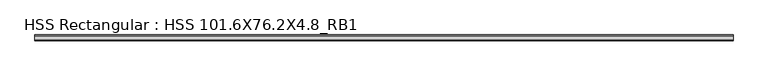
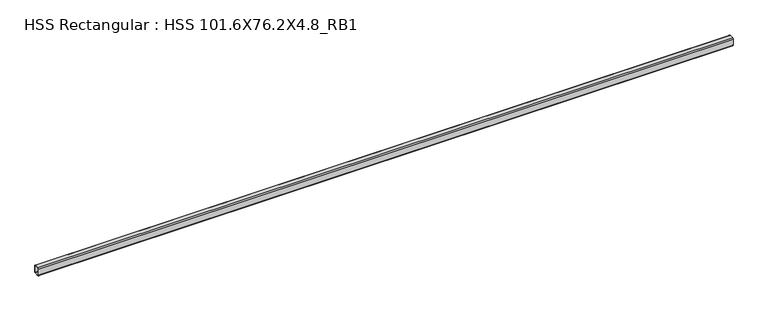
"""IFC4 building model written with IfcOpenShell, lengths in millimetres: beam geometry, HSS Rectangular : HSS 101.6X76.2X4.8_RB1."""

import ifcopenshell
import ifcopenshell.guid

model = None  # the IFC model being written
_history = None  # IfcOwnerHistory: only IFC2X3 demands one
_inside = {}  # id of a spatial element -> (the spatial element, [elements in it])
_under = {}  # id of a project, library or spatial element -> (it, [spatial elements below it])
_declared = {}  # id of a project -> (the project, [libraries it declares])
_typed = {}  # id of a type object -> (the type object, [elements of that type])
_made_of = {}  # id of a material, layer set ... -> (it, [elements and type objects made of it])


def new_model(schema):
    """Start an empty IFC model of exactly this schema.

    Asked for "IFC4X3", IfcOpenShell would pick the latest addendum, in which some entities
    have other attributes; the version numbers below select the first issue.
    IFC2X3 requires an IfcOwnerHistory on every rooted entity: one is made here for all.
    """
    global model, _history
    if schema == "IFC4X3":
        model = ifcopenshell.file(schema_version=(4, 3, 0, 0))
    else:
        model = ifcopenshell.file(schema=schema)
    _inside.clear()
    _under.clear()
    _declared.clear()
    _typed.clear()
    _made_of.clear()
    _history = None
    if model.schema == "IFC2X3":
        org = make("IfcOrganization", Name="unknown")
        user = make(
            "IfcPersonAndOrganization",
            ThePerson=make("IfcPerson", FamilyName="unknown"),
            TheOrganization=org,
        )
        app = make(
            "IfcApplication",
            ApplicationDeveloper=org,
            Version="unknown",
            ApplicationFullName="unknown",
            ApplicationIdentifier="unknown",
        )
        _history = make(
            "IfcOwnerHistory",
            OwningUser=user,
            OwningApplication=app,
            ChangeAction="ADDED",
            CreationDate=0,
        )
    return model


def make(cls, **values):
    """One entity of the class cls with the attributes given. An attribute that is None is left unset."""
    return model.create_entity(
        cls, **{name: value for name, value in values.items() if value is not None}
    )


def rooted(cls, **values):
    """An entity with a GlobalId (a new one), such as an element, a storey or a relation."""
    return make(cls, GlobalId=ifcopenshell.guid.new(), OwnerHistory=_history, **values)


def si_unit(unit_type, name, prefix=None):
    """IfcSIUnit, for example si_unit("LENGTHUNIT", "METRE", prefix="MILLI")."""
    return make("IfcSIUnit", UnitType=unit_type, Prefix=prefix, Name=name)


def assignment(units):
    """IfcUnitAssignment: the units of a project."""
    return None if units is None else make("IfcUnitAssignment", Units=units)


def point(xyz):
    """IfcCartesianPoint."""
    return None if xyz is None else make("IfcCartesianPoint", Coordinates=xyz)


def direction(xyz):
    """IfcDirection."""
    return None if xyz is None else make("IfcDirection", DirectionRatios=xyz)


def frame(location, z_axis=None, x_axis=None):
    """IfcAxis2Placement3D, a coordinate frame: its origin and axes. An axis left out is left unset."""
    return make(
        "IfcAxis2Placement3D",
        Location=point(location),
        Axis=direction(z_axis),
        RefDirection=direction(x_axis),
    )


def frame_2d(location, x_axis=None):
    """IfcAxis2Placement2D, a coordinate frame in the plane: its origin and x axis."""
    return make(
        "IfcAxis2Placement2D", Location=point(location), RefDirection=direction(x_axis)
    )


def origin():
    """The frame at (0, 0, 0) with its axes left unset."""
    return frame((0.0, 0.0, 0.0))


def place(relative_to, where):
    """IfcLocalPlacement: puts the frame where relative to a parent placement (None: the world)."""
    return make(
        "IfcLocalPlacement", PlacementRelTo=relative_to, RelativePlacement=where
    )


def context(
    kind, dimensions, precision=None, world=None, true_north=None, identifier=None
):
    """IfcGeometricRepresentationContext, for example the 3D "Model" context."""
    return make(
        "IfcGeometricRepresentationContext",
        ContextIdentifier=identifier,
        ContextType=kind,
        CoordinateSpaceDimension=dimensions,
        Precision=precision,
        WorldCoordinateSystem=world,
        TrueNorth=true_north,
    )


def project(units=None, contexts=None):
    """IfcProject with its units and contexts."""
    return rooted(
        "IfcProject",
        Name="project",
        RepresentationContexts=contexts,
        UnitsInContext=assignment(units),
    )


def spatial(cls, under=None, at=None, **own):
    """A site, building, storey or space (cls), placed at a placement, below another one or the project."""
    s = rooted(cls, ObjectPlacement=at, **own)
    if under is not None:
        _under.setdefault(under.id(), (under, []))[1].append(s)
    return s


def polyline(points):
    """IfcPolyline through the points."""
    return make("IfcPolyline", Points=[point(p) for p in points])


def circle_curve(where, radius):
    """IfcCircle in the frame where."""
    return make("IfcCircle", Position=where, Radius=radius)


def trimmed(basis, trim1, trim2, sense, master):
    """IfcTrimmedCurve: the piece of a basis curve between two trims."""
    return make(
        "IfcTrimmedCurve",
        BasisCurve=basis,
        Trim1=trim1,
        Trim2=trim2,
        SenseAgreement=sense,
        MasterRepresentation=master,
    )


def segment(curve, same_sense, transition):
    """IfcCompositeCurveSegment."""
    return make(
        "IfcCompositeCurveSegment",
        Transition=transition,
        SameSense=same_sense,
        ParentCurve=curve,
    )


def composite_curve(segments, self_intersect=None):
    """IfcCompositeCurve: segments joined end to end."""
    return make("IfcCompositeCurve", Segments=segments, SelfIntersect=self_intersect)


def outline(outer, holes=None, kind="AREA"):
    """IfcArbitraryClosedProfileDef: a profile drawn as a closed curve; with holes, ...WithVoids."""
    if holes is None:
        return make("IfcArbitraryClosedProfileDef", ProfileType=kind, OuterCurve=outer)
    return make(
        "IfcArbitraryProfileDefWithVoids",
        ProfileType=kind,
        OuterCurve=outer,
        InnerCurves=holes,
    )


def extrude(swept, where, along, depth):
    """IfcExtrudedAreaSolid: the profile swept, set in the frame where, extruded along a direction by depth."""
    return make(
        "IfcExtrudedAreaSolid",
        SweptArea=swept,
        Position=where,
        ExtrudedDirection=direction(along),
        Depth=depth,
    )


def shape(context_of_items, identifier, shape_type, items):
    """IfcShapeRepresentation: the items that make up one representation, for example the "Body"."""
    return make(
        "IfcShapeRepresentation",
        ContextOfItems=context_of_items,
        RepresentationIdentifier=identifier,
        RepresentationType=shape_type,
        Items=items,
    )


def source(mapping_origin, context_of_items, identifier, shape_type, items):
    """IfcRepresentationMap: a shape defined once, which mapped items show again and again."""
    return make(
        "IfcRepresentationMap",
        MappingOrigin=mapping_origin,
        MappedRepresentation=shape(context_of_items, identifier, shape_type, items),
    )


def transform(
    local_origin,
    x_axis=None,
    y_axis=None,
    z_axis=None,
    scale=None,
    scale2=None,
    scale3=None,
    uniform=True,
):
    """IfcCartesianTransformationOperator3D, or its non-uniform kind. x_axis, y_axis, z_axis: its Axis1, 2, 3."""
    if uniform:
        return make(
            "IfcCartesianTransformationOperator3D",
            Axis1=direction(x_axis),
            Axis2=direction(y_axis),
            LocalOrigin=point(local_origin),
            Scale=scale,
            Axis3=direction(z_axis),
        )
    return make(
        "IfcCartesianTransformationOperator3DnonUniform",
        Axis1=direction(x_axis),
        Axis2=direction(y_axis),
        LocalOrigin=point(local_origin),
        Scale=scale,
        Axis3=direction(z_axis),
        Scale2=scale2,
        Scale3=scale3,
    )


def mapped(mapping_source, mapping_target):
    """IfcMappedItem: shows the shape of a source again, moved by a transform."""
    return make(
        "IfcMappedItem", MappingSource=mapping_source, MappingTarget=mapping_target
    )


def made_of(thing, what):
    """Note that an element or type object is made of a material, layer set ...; save() writes the relation."""
    if what is not None:
        _made_of.setdefault(what.id(), (what, []))[1].append(thing)
    return thing


def element(
    cls,
    number,
    at=None,
    inside=None,
    cuts=None,
    type_object=None,
    material=None,
    context=None,
    identifier="Body",
    shape_type=None,
    held_by="IfcProductDefinitionShape",
    body=None,
    shapes=None,
    **own,
):
    """One element of the class cls, such as IfcWall. Its Tag is "e" and its number.

    at: its placement. inside: the storey or other place that contains it. cuts: it is an
    opening in that element (IfcRelVoidsElement). A single representation is given by context,
    identifier, shape_type and body (its items); several are given by shapes. held_by: the class
    of the entity that holds the representations. save() writes the other relations.
    """
    e = rooted(cls, Tag="e%d" % number, ObjectPlacement=at, **own)
    if body is not None:
        shapes = [shape(context, identifier, shape_type, body)]
    if shapes is not None:
        e.Representation = make(held_by, Representations=shapes)
    if inside is not None:
        _inside.setdefault(inside.id(), (inside, []))[1].append(e)
    if cuts is not None:
        rooted(
            "IfcRelVoidsElement", RelatingBuildingElement=cuts, RelatedOpeningElement=e
        )
    if type_object is not None:
        _typed.setdefault(type_object.id(), (type_object, []))[1].append(e)
    return made_of(e, material)


def aggregate(whole, parts):
    """IfcRelAggregates: a whole, such as a stair, and the parts it consists of."""
    return rooted("IfcRelAggregates", RelatingObject=whole, RelatedObjects=parts)


def save(model, path):
    """Write the relations noted so far, then the file.

    IfcRelAggregates (storeys below a building ...), IfcRelContainedInSpatialStructure (elements
    in a storey), IfcRelDefinesByType, IfcRelAssociatesMaterial and IfcRelDeclares: one each for
    every whole, place, type object, material and project.
    """
    for whole, parts in _under.values():
        aggregate(whole, parts)
    for where, things in _inside.values():
        rooted(
            "IfcRelContainedInSpatialStructure",
            RelatedElements=things,
            RelatingStructure=where,
        )
    for kind, things in _typed.values():
        rooted("IfcRelDefinesByType", RelatedObjects=things, RelatingType=kind)
    for what, things in _made_of.values():
        rooted("IfcRelAssociatesMaterial", RelatedObjects=things, RelatingMaterial=what)
    for by, libraries in _declared.values():
        rooted("IfcRelDeclares", RelatingContext=by, RelatedDefinitions=libraries)
    model.write(path)


def hss_rectangular_hss_101_6x76_2x4_8_rb1_0e89a898(model_context):
    return source(origin(), model_context, "Body", "SweptSolid", [
        extrude(outline(composite_curve([segment(polyline([(38.1, 41.275), (38.1, -41.275)]), True, "CONTINUOUS"), segment(trimmed(circle_curve(frame_2d((28.575, -41.275)), 9.525), [point((38.1, -41.275))], [point((28.575, -50.8))], False, "CARTESIAN"), True, "CONTINUOUS"), segment(polyline([(28.575, -50.8), (-28.575, -50.8)]), True, "CONTINUOUS"), segment(trimmed(circle_curve(frame_2d((-28.575, -41.275)), 9.525), [point((-28.575, -50.8))], [point((-38.1, -41.275))], False, "CARTESIAN"), True, "CONTINUOUS"), segment(polyline([(-38.1, -41.275), (-38.1, 41.275)]), True, "CONTINUOUS"), segment(trimmed(circle_curve(frame_2d((-28.575, 41.275)), 9.525), [point((-38.1, 41.275))], [point((-28.575, 50.8))], False, "CARTESIAN"), True, "CONTINUOUS"), segment(polyline([(-28.575, 50.8), (28.575, 50.8)]), True, "CONTINUOUS"), segment(trimmed(circle_curve(frame_2d((28.575, 41.275)), 9.525), [point((28.575, 50.8))], [point((38.1, 41.275))], False, "CARTESIAN"), True, "CONTINUOUS")], self_intersect=False), holes=[composite_curve([segment(trimmed(circle_curve(frame_2d((-28.575, 41.275)), 4.7625), [point((-28.575, 46.0375))], [point((-33.3375, 41.275))], True, "CARTESIAN"), True, "CONTINUOUS"), segment(polyline([(-33.3375, 41.275), (-33.3375, -41.275)]), True, "CONTINUOUS"), segment(trimmed(circle_curve(frame_2d((-28.575, -41.275)), 4.7625), [point((-33.3375, -41.275))], [point((-28.575, -46.0375))], True, "CARTESIAN"), True, "CONTINUOUS"), segment(polyline([(-28.575, -46.0375), (28.575, -46.0375)]), True, "CONTINUOUS"), segment(trimmed(circle_curve(frame_2d((28.575, -41.275)), 4.7625), [point((28.575, -46.0375))], [point((33.3375, -41.275))], True, "CARTESIAN"), True, "CONTINUOUS"), segment(polyline([(33.3375, -41.275), (33.3375, 41.275)]), True, "CONTINUOUS"), segment(trimmed(circle_curve(frame_2d((28.575, 41.275)), 4.7625), [point((33.3375, 41.275))], [point((28.575, 46.0375))], True, "CARTESIAN"), True, "CONTINUOUS"), segment(polyline([(28.575, 46.0375), (-28.575, 46.0375)]), True, "CONTINUOUS")], self_intersect=False)]), frame((1636.9347881, 0.0, 0.0), z_axis=(1.0, 0.0, 0.0), x_axis=(0.0, 1.0, 0.0)), (0.0, 0.0, 1.0), 8849.9633079),
    ])


if __name__ == "__main__":
    model = new_model("IFC4")
    model_context = context("Model", 3, world=origin())
    ifc_project = project(units=[si_unit("LENGTHUNIT", "METRE", prefix="MILLI")], contexts=[model_context])
    site = spatial("IfcSite", under=ifc_project)
    building = spatial("IfcBuilding", under=site)
    placement = place(None, origin())
    hss_rectangular_hss_101_6x76_2x4_8_rb1_shape = hss_rectangular_hss_101_6x76_2x4_8_rb1_0e89a898(model_context)
    element("IfcBeam", 1, ObjectType="HSS Rectangular : HSS 101.6X76.2X4.8_RB1", at=placement, inside=building, context=model_context, shape_type="MappedRepresentation", body=[
        mapped(hss_rectangular_hss_101_6x76_2x4_8_rb1_shape, transform((0.0, 0.0, 0.0), x_axis=(1.0, 0.0, 0.0), y_axis=(0.0, 1.0, 0.0), z_axis=(0.0, 0.0, 1.0))),
    ])
    save(model, "model.ifc")

# Revit data of these elements
# Type "HSS Rectangular : HSS 101.6X76.2X4.8_RB1"
#   Section Name Key = "HSS 4X3X3/16"
#   Assembly Code = "B10"
#   Width = 7.62 cm
#   Wall Nominal Thickness = 0.4763 cm
#   Wall Design Thickness = 0.442 cm
#   Torsional Moment of Inertia = 260.561 cm⁴
#   Torsional Modulus = 61.2876 cm³
#   Section Area = 14.4516 cm²
#   Plastic Modulus weak axis = 40.3122 cm³
#   Plastic Modulus strong axis = 49.1612 cm³
#   Perimeter = 0.881482 m²/m
#   Outer Fillet = 0.9525 cm
#   Nominal Weight = 12.1285 kgf/m
#   Moment of Inertia weak axis = 131.529 cm⁴
#   Moment of Inertia strong axis = 205.202 cm⁴
#   Inner Fillet = 0.4763 cm
#   Height = 10.16 cm
#   Elastic Modulus weak axis = 34.4128 cm³
#   Elastic Modulus strong axis = 40.476 cm³
#   Centroid Vertical = 5.08 cm
#   Centroid Horizontal = 3.81 cm
#   Length [instance default] = 1524 mm
#   Structural Material [instance default] = Steel ASTM A500, Grade B, Rectangular and Square
#   Principal Axes Angle = 0
# Element 1 (IfcBeam, "HSS Rectangular : HSS 101.6X76.2X4.8_RB1")
#   Structural Material = Steel ASTM A992
#   Materials on its faces: "Steel ASTM A992"
# Materials
#   "Steel ASTM A500, Grade B, Rectangular and Square": class "Metal", colour RGB 199 199 199, transparency 0, Description = "Carbon steel", Cost = 0
#   "Steel ASTM A992": class "Metal", colour RGB 199 199 199, transparency 0, Description = "Structural steel 50ksi", Cost = 0
